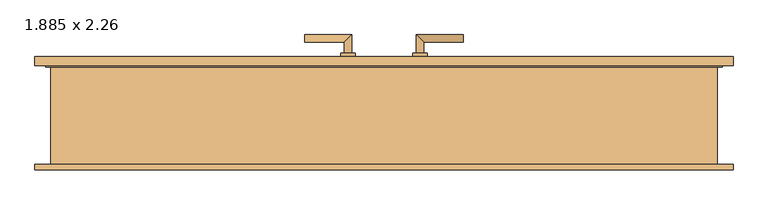
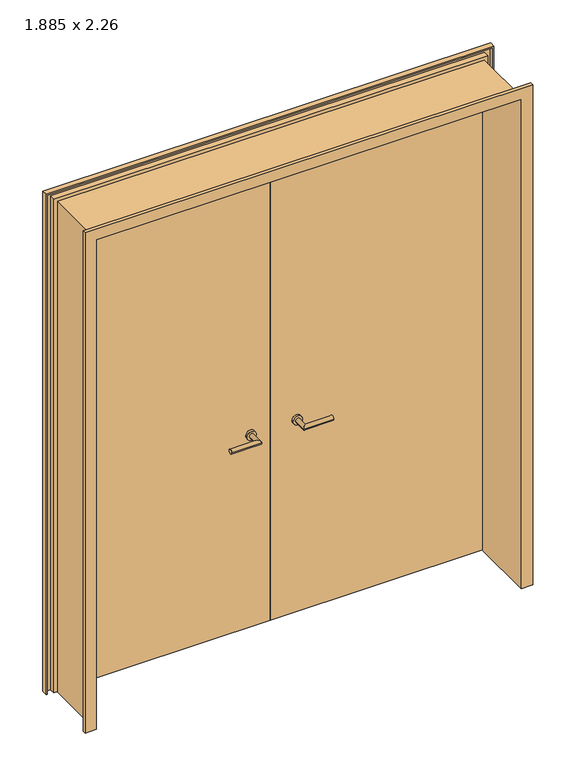
"""IFC4 building model written with IfcOpenShell, lengths in millimetres: door geometry, Drehflügel 2-flg - Stahlzarge : 1.885 x 2.26."""

from ifc_helpers import new_model, si_unit, point, frame, frame_2d, origin, place, context, project, spatial, polyline, circle_curve, ellipse_curve, trimmed, segment, composite_curve, outline, extrude, faceted_brep, source, transform, mapped, element, save
from ifc_brep_helpers import plane_surface, cylinder_surface, advanced_brep


def door_1_885_x_2_26_ea08af73(model_context):
    return source(origin(), model_context, "Body", "SolidModel", [
        advanced_brep(
        [(-90.0, 126.9346141, 1000.0), (-110.0, 126.9346141, 1000.0), (-110.0, 76.9346141, 1000.0), (-90.0, 56.9346141, 1000.0), (-220.0, 56.9346141, 1000.0), (-220.0, 76.9346141, 1000.0)],
        [
            (0, 1, circle_curve(frame((-100.0, 126.9346141, 1000.0), z_axis=(0.0, 1.0, 0.0), x_axis=(-1.0, 0.0, 0.0)), 10.0)),
            (1, 0, circle_curve(frame((-100.0, 126.9346141, 1000.0), z_axis=(0.0, 1.0, 0.0), x_axis=(-1.0, 0.0, 0.0)), 10.0)),
            (1, 2),
            (2, 3, ellipse_curve(frame((-100.0, 66.9346141, 1000.0), z_axis=(0.7071067811865385, 0.7071067811865565, 0.0), x_axis=(-0.7071067811865563, 0.7071067811865386, 0.0)), 14.1421356, 10.0)),
            (3, 0),
            (3, 2, ellipse_curve(frame((-100.0, 66.9346141, 1000.0), z_axis=(0.7071067811865385, 0.7071067811865565, 0.0), x_axis=(-0.7071067811865563, 0.7071067811865386, 0.0)), 14.1421356, 10.0)),
            (4, 5, circle_curve(frame((-220.0, 66.9346141, 1000.0), z_axis=(-1.0, 0.0, 0.0), x_axis=(0.0, 1.0, 0.0)), 10.0)),
            (5, 4, circle_curve(frame((-220.0, 66.9346141, 1000.0), z_axis=(-1.0, 0.0, 0.0), x_axis=(0.0, 1.0, 0.0)), 10.0)),
            (2, 5),
            (4, 3),
        ],
        [
            plane_surface(frame((-100.0, 126.9346141, -287.7526403), z_axis=(0.0, 1.0, 0.0), x_axis=(0.0, 0.0, 1.0))),
            cylinder_surface(frame((-100.0, 126.9346141, 1000.0), z_axis=(0.0, 1.0, 0.0), x_axis=(-1.0, 0.0, 0.0)), 10.0),
            plane_surface(frame((-220.0, 66.9346141, -287.7526403), z_axis=(-1.0, 0.0, 0.0), x_axis=(0.0, 0.0, 1.0))),
            cylinder_surface(frame((-100.0, 66.9346141, 1000.0), z_axis=(1.0, 0.0, 0.0), x_axis=(0.0, 1.0, 0.0)), 10.0),
        ],
        [
            (0, [[1, 2]]),
            (1, [[3, 4, 5, -2]]),
            (1, [[-5, 6, -3, -1]]),
            (2, [[7, 8]]),
            (3, [[9, -7, 10, -4]]),
            (3, [[-10, -8, -9, -6]]),
        ],
    ),
        advanced_brep(
        [(-110.0, 186.9346141, 1000.0), (-90.0, 186.9346141, 1000.0), (-90.0, 236.9346141, 1000.0), (-110.0, 216.9346141, 1000.0), (-220.0, 216.9346141, 1000.0), (-220.0, 236.9346141, 1000.0)],
        [
            (0, 1, circle_curve(frame((-100.0, 186.9346141, 1000.0), z_axis=(0.0, -1.0, 0.0), x_axis=(1.0, 0.0, 0.0)), 10.0)),
            (1, 0, circle_curve(frame((-100.0, 186.9346141, 1000.0), z_axis=(0.0, -1.0, 0.0), x_axis=(1.0, 0.0, 0.0)), 10.0)),
            (1, 2),
            (2, 3, ellipse_curve(frame((-100.0, 226.9346141, 1000.0), z_axis=(0.7071067811865475, -0.7071067811865475, 0.0), x_axis=(-0.7071067811865474, -0.7071067811865476, 0.0)), 14.1421356, 10.0)),
            (3, 0),
            (3, 2, ellipse_curve(frame((-100.0, 226.9346141, 1000.0), z_axis=(0.7071067811865475, -0.7071067811865475, 0.0), x_axis=(-0.7071067811865474, -0.7071067811865476, 0.0)), 14.1421356, 10.0)),
            (4, 5, circle_curve(frame((-220.0, 226.9346141, 1000.0), z_axis=(-1.0, 0.0, 0.0), x_axis=(0.0, 1.0, 0.0)), 10.0)),
            (5, 4, circle_curve(frame((-220.0, 226.9346141, 1000.0), z_axis=(-1.0, 0.0, 0.0), x_axis=(0.0, 1.0, 0.0)), 10.0)),
            (2, 5),
            (4, 3),
        ],
        [
            plane_surface(frame((-100.0, 186.9346141, -287.7526403), z_axis=(0.0, -1.0, 0.0), x_axis=(0.0, 0.0, 1.0))),
            cylinder_surface(frame((-100.0, 186.9346141, 1000.0), z_axis=(0.0, -1.0, 0.0), x_axis=(1.0, 0.0, 0.0)), 10.0),
            plane_surface(frame((-220.0, 226.9346141, -287.7526403), z_axis=(-1.0, 0.0, 0.0), x_axis=(0.0, 0.0, 1.0))),
            cylinder_surface(frame((-100.0, 226.9346141, 1000.0), z_axis=(1.0, 0.0, 0.0), x_axis=(0.0, 1.0, 0.0)), 10.0),
        ],
        [
            (0, [[1, 2]]),
            (1, [[3, 4, 5, -2]]),
            (1, [[-5, 6, -3, -1]]),
            (2, [[7, 8]]),
            (3, [[9, -7, 10, -4]]),
            (3, [[-10, -8, -9, -6]]),
        ],
    ),
        extrude(outline(composite_curve([segment(trimmed(circle_curve(frame_2d((1000.0, -100.0)), 20.0), [point((1000.0, -80.0))], [point((1000.0, -120.0))], False, "CARTESIAN"), True, "CONTINUOUS"), segment(trimmed(circle_curve(frame_2d((1000.0, -100.0)), 20.0), [point((1000.0, -120.0))], [point((1000.0, -80.0))], False, "CARTESIAN"), True, "CONTINUOUS")], self_intersect=False)), frame((0.0, 116.9346141, 0.0), z_axis=(0.0, 1.0, 0.0), x_axis=(0.0, 0.0, 1.0)), (0.0, 0.0, 1.0), 10.0),
        extrude(outline(composite_curve([segment(trimmed(circle_curve(frame_2d((1000.0, -100.0)), 20.0), [point((1000.0, -80.0))], [point((1000.0, -120.0))], False, "CARTESIAN"), True, "CONTINUOUS"), segment(trimmed(circle_curve(frame_2d((1000.0, -100.0)), 20.0), [point((1000.0, -120.0))], [point((1000.0, -80.0))], False, "CARTESIAN"), True, "CONTINUOUS")], self_intersect=False)), frame((0.0, 176.9346141, 0.0), z_axis=(0.0, 1.0, 0.0), x_axis=(0.0, 0.0, 1.0)), (0.0, 0.0, 1.0), 10.0),
        advanced_brep(
        [(90.0, 126.9346141, 1000.0), (110.0, 126.9346141, 1000.0), (90.0, 56.9346141, 1000.0), (110.0, 76.9346141, 1000.0), (220.0, 56.9346141, 1000.0), (220.0, 76.9346141, 1000.0)],
        [
            (0, 1, circle_curve(frame((100.0, 126.9346141, 1000.0), z_axis=(0.0, 1.0, 0.0), x_axis=(1.0, 0.0, 0.0)), 10.0)),
            (1, 0, circle_curve(frame((100.0, 126.9346141, 1000.0), z_axis=(0.0, 1.0, 0.0), x_axis=(1.0, 0.0, 0.0)), 10.0)),
            (0, 2),
            (2, 3, ellipse_curve(frame((100.0, 66.9346141, 1000.0), z_axis=(-0.7071067811865385, 0.7071067811865565, 0.0), x_axis=(0.7071067811865563, 0.7071067811865386, 0.0)), 14.1421356, 10.0)),
            (3, 1),
            (3, 2, ellipse_curve(frame((100.0, 66.9346141, 1000.0), z_axis=(-0.7071067811865385, 0.7071067811865565, 0.0), x_axis=(0.7071067811865563, 0.7071067811865386, 0.0)), 14.1421356, 10.0)),
            (4, 5, circle_curve(frame((220.0, 66.9346141, 1000.0), z_axis=(1.0, 0.0, 0.0), x_axis=(0.0, 1.0, 0.0)), 10.0)),
            (5, 4, circle_curve(frame((220.0, 66.9346141, 1000.0), z_axis=(1.0, 0.0, 0.0), x_axis=(0.0, 1.0, 0.0)), 10.0)),
            (2, 4),
            (5, 3),
        ],
        [
            plane_surface(frame((100.0, 126.9346141, -287.7526403), z_axis=(0.0, 1.0, 0.0), x_axis=(0.0, 0.0, 1.0))),
            cylinder_surface(frame((100.0, 126.9346141, 1000.0), z_axis=(0.0, 1.0, 0.0), x_axis=(1.0, 0.0, 0.0)), 10.0),
            plane_surface(frame((220.0, 66.9346141, -287.7526403), z_axis=(1.0, 0.0, 0.0), x_axis=(0.0, 0.0, 1.0))),
            cylinder_surface(frame((100.0, 66.9346141, 1000.0), z_axis=(-1.0, 0.0, 0.0), x_axis=(0.0, 1.0, 0.0)), 10.0),
        ],
        [
            (0, [[1, 2]]),
            (1, [[-1, 3, 4, 5]]),
            (1, [[-2, -5, 6, -3]]),
            (2, [[7, 8]]),
            (3, [[-4, 9, -8, 10]]),
            (3, [[-6, -10, -7, -9]]),
        ],
    ),
        advanced_brep(
        [(110.0, 186.9346141, 1000.0), (90.0, 186.9346141, 1000.0), (110.0, 216.9346141, 1000.0), (90.0, 236.9346141, 1000.0), (220.0, 216.9346141, 1000.0), (220.0, 236.9346141, 1000.0)],
        [
            (0, 1, circle_curve(frame((100.0, 186.9346141, 1000.0), z_axis=(0.0, -1.0, 0.0), x_axis=(-1.0, 0.0, 0.0)), 10.0)),
            (1, 0, circle_curve(frame((100.0, 186.9346141, 1000.0), z_axis=(0.0, -1.0, 0.0), x_axis=(-1.0, 0.0, 0.0)), 10.0)),
            (0, 2),
            (2, 3, ellipse_curve(frame((100.0, 226.9346141, 1000.0), z_axis=(-0.7071067811865475, -0.7071067811865475, 0.0), x_axis=(0.7071067811865474, -0.7071067811865476, 0.0)), 14.1421356, 10.0)),
            (3, 1),
            (3, 2, ellipse_curve(frame((100.0, 226.9346141, 1000.0), z_axis=(-0.7071067811865475, -0.7071067811865475, 0.0), x_axis=(0.7071067811865474, -0.7071067811865476, 0.0)), 14.1421356, 10.0)),
            (4, 5, circle_curve(frame((220.0, 226.9346141, 1000.0), z_axis=(1.0, 0.0, 0.0), x_axis=(0.0, 1.0, 0.0)), 10.0)),
            (5, 4, circle_curve(frame((220.0, 226.9346141, 1000.0), z_axis=(1.0, 0.0, 0.0), x_axis=(0.0, 1.0, 0.0)), 10.0)),
            (2, 4),
            (5, 3),
        ],
        [
            plane_surface(frame((100.0, 186.9346141, -287.7526403), z_axis=(0.0, -1.0, 0.0), x_axis=(0.0, 0.0, 1.0))),
            cylinder_surface(frame((100.0, 186.9346141, 1000.0), z_axis=(0.0, -1.0, 0.0), x_axis=(-1.0, 0.0, 0.0)), 10.0),
            plane_surface(frame((220.0, 226.9346141, -287.7526403), z_axis=(1.0, 0.0, 0.0), x_axis=(0.0, 0.0, 1.0))),
            cylinder_surface(frame((100.0, 226.9346141, 1000.0), z_axis=(-1.0, 0.0, 0.0), x_axis=(0.0, 1.0, 0.0)), 10.0),
        ],
        [
            (0, [[1, 2]]),
            (1, [[-1, 3, 4, 5]]),
            (1, [[-2, -5, 6, -3]]),
            (2, [[7, 8]]),
            (3, [[-4, 9, -8, 10]]),
            (3, [[-6, -10, -7, -9]]),
        ],
    ),
        extrude(outline(composite_curve([segment(trimmed(circle_curve(frame_2d((1000.0, 100.0)), 20.0), [point((1000.0, 80.0))], [point((1000.0, 120.0))], False, "CARTESIAN"), True, "CONTINUOUS"), segment(trimmed(circle_curve(frame_2d((1000.0, 100.0)), 20.0), [point((1000.0, 120.0))], [point((1000.0, 80.0))], False, "CARTESIAN"), True, "CONTINUOUS")], self_intersect=False)), frame((0.0, 116.9346141, 0.0), z_axis=(0.0, 1.0, 0.0), x_axis=(0.0, 0.0, 1.0)), (0.0, 0.0, 1.0), 10.0),
        extrude(outline(composite_curve([segment(trimmed(circle_curve(frame_2d((1000.0, 100.0)), 20.0), [point((1000.0, 80.0))], [point((1000.0, 120.0))], False, "CARTESIAN"), True, "CONTINUOUS"), segment(trimmed(circle_curve(frame_2d((1000.0, 100.0)), 20.0), [point((1000.0, 120.0))], [point((1000.0, 80.0))], False, "CARTESIAN"), True, "CONTINUOUS")], self_intersect=False)), frame((0.0, 176.9346141, 0.0), z_axis=(0.0, 1.0, 0.0), x_axis=(0.0, 0.0, 1.0)), (0.0, 0.0, 1.0), 10.0),
        extrude(outline(polyline([(0.0, 151.9346141), (-932.5, 151.9346141), (-932.5, 176.9346141), (0.0, 176.9346141), (0.0, 151.9346141)])), frame((0.0, 0.0, 100.0), z_axis=(0.0, 0.0, 1.0), x_axis=(1.0, 0.0, 0.0)), (0.0, 0.0, 1.0), 2250.0),
        extrude(outline(polyline([(932.5, 151.9346141), (0.0, 151.9346141), (0.0, 176.9346141), (932.5, 176.9346141), (932.5, 151.9346141)])), frame((0.0, 0.0, 100.0), z_axis=(0.0, 0.0, 1.0), x_axis=(1.0, 0.0, 0.0)), (0.0, 0.0, 1.0), 2250.0),
        faceted_brep([(967.0, -138.0653859, 100.0), (917.5, -138.0653859, 100.0), (917.5, 151.9346141, 100.0), (932.5, 151.9346141, 100.0), (932.5, 176.9346141, 100.0), (967.0, 176.9346141, 100.0), (967.0, 151.9346141, 100.0), (962.0, 151.9346141, 100.0), (962.0, 171.9346141, 100.0), (937.5, 171.9346141, 100.0), (937.5, 146.9346141, 100.0), (922.5, 146.9346141, 100.0), (922.5, -133.0653859, 100.0), (962.0, -133.0653859, 100.0), (962.0, -123.0653859, 100.0), (967.0, -123.0653859, 100.0), (967.0, -138.0653859, 2384.5), (-967.0, -138.0653859, 2384.5), (-967.0, -138.0653859, 100.0), (-917.5, -138.0653859, 100.0), (-917.5, -138.0653859, 2335.0), (917.5, -138.0653859, 2335.0), (917.5, 151.9346141, 2335.0), (-917.5, 151.9346141, 2335.0), (-917.5, 151.9346141, 100.0), (-932.5, 151.9346141, 100.0), (-932.5, 151.9346141, 2350.0), (932.5, 151.9346141, 2350.0), (932.5, 176.9346141, 2350.0), (-932.5, 176.9346141, 2350.0), (-932.5, 176.9346141, 100.0), (-967.0, 176.9346141, 100.0), (-967.0, 176.9346141, 2384.5), (967.0, 176.9346141, 2384.5), (967.0, 151.9346141, 2384.5), (-967.0, 151.9346141, 2384.5), (-967.0, 151.9346141, 100.0), (-962.0, 151.9346141, 100.0), (-962.0, 151.9346141, 2379.5), (962.0, 151.9346141, 2379.5), (962.0, 171.9346141, 2379.5), (-962.0, 171.9346141, 2379.5), (-962.0, 171.9346141, 100.0), (-937.5, 171.9346141, 100.0), (-937.5, 171.9346141, 2355.0), (937.5, 171.9346141, 2355.0), (937.5, 146.9346141, 2355.0), (-937.5, 146.9346141, 2355.0), (-937.5, 146.9346141, 100.0), (-922.5, 146.9346141, 100.0), (-922.5, 146.9346141, 2340.0), (922.5, 146.9346141, 2340.0), (922.5, -133.0653859, 2340.0), (-922.5, -133.0653859, 2340.0), (-922.5, -133.0653859, 100.0), (-962.0, -133.0653859, 100.0), (-962.0, -133.0653859, 2379.5), (962.0, -133.0653859, 2379.5), (962.0, -123.0653859, 2379.5), (-962.0, -123.0653859, 2379.5), (-962.0, -123.0653859, 100.0), (-967.0, -123.0653859, 100.0), (-967.0, -123.0653859, 2384.5), (967.0, -123.0653859, 2384.5)], [[[0, 1, 2, 3, 4, 5, 6, 7, 8, 9, 10, 11, 12, 13, 14, 15]], [[1, 0, 16, 17, 18, 19, 20, 21]], [[2, 1, 21, 22]], [[3, 2, 22, 23, 24, 25, 26, 27]], [[4, 3, 27, 28]], [[5, 4, 28, 29, 30, 31, 32, 33]], [[6, 5, 33, 34]], [[7, 6, 34, 35, 36, 37, 38, 39]], [[8, 7, 39, 40]], [[9, 8, 40, 41, 42, 43, 44, 45]], [[10, 9, 45, 46]], [[11, 10, 46, 47, 48, 49, 50, 51]], [[12, 11, 51, 52]], [[13, 12, 52, 53, 54, 55, 56, 57]], [[14, 13, 57, 58]], [[15, 14, 58, 59, 60, 61, 62, 63]], [[0, 15, 63, 16]], [[17, 62, 61, 18]], [[18, 61, 60, 55, 54, 49, 48, 43, 42, 37, 36, 31, 30, 25, 24, 19]], [[23, 20, 19, 24]], [[29, 26, 25, 30]], [[35, 32, 31, 36]], [[41, 38, 37, 42]], [[47, 44, 43, 48]], [[53, 50, 49, 54]], [[59, 56, 55, 60]], [[22, 21, 20, 23]], [[28, 27, 26, 29]], [[34, 33, 32, 35]], [[40, 39, 38, 41]], [[46, 45, 44, 47]], [[52, 51, 50, 53]], [[58, 57, 56, 59]], [[16, 63, 62, 17]]]),
    ])


if __name__ == "__main__":
    model = new_model("IFC4")
    model_context = context("Model", 3, world=origin())
    ifc_project = project(units=[si_unit("LENGTHUNIT", "METRE", prefix="MILLI")], contexts=[model_context])
    site = spatial("IfcSite", under=ifc_project)
    building = spatial("IfcBuilding", under=site)
    placement = place(None, origin())
    door_1_885_x_2_26_shape = door_1_885_x_2_26_ea08af73(model_context)
    element("IfcDoor", 1, ObjectType="Drehflügel 2-flg - Stahlzarge : 1.885 x 2.26", at=placement, inside=building, context=model_context, shape_type="MappedRepresentation", body=[
        mapped(door_1_885_x_2_26_shape, transform((0.0, 0.0, 0.0), x_axis=(1.0, 0.0, 0.0), y_axis=(0.0, 1.0, 0.0), z_axis=(0.0, 0.0, 1.0))),
    ])
    save(model, "model.ifc")

# Revit data of these elements
# Type "Drehflügel 2-flg - Stahlzarge : 1.885 x 2.26"
#   Construction Type Id = "DOOR"
#   Type Mark = "19"
#   Operation = "DoubleDoorSingleSwing"
#   Keynote = "16.03"
#   Analytic Construction = "Hölzern"
#   Thermal Resistance (R) = 0.270117 (m²·K)/W
#   Heat Transfer Coefficient (U) = 2.1944 W/(m²·K)
#   Rough Width = 1.885 m
#   Rough Height [instance default] = 2.360 m
#   Höhe Türgriff = 0.900 m
#   Height = 2.260 m
#   Fußbodenaufbau [instance default] = 0.100 m
#   Width = 1.885 m
#   Sichtbarkeit Sturzlinien [instance default] = yes
#   Türgriff auswählen [instance default] = element 219327
#   Türgriff [instance default] = none
#   Türflügel [instance default] = none
#   Rahmen/Pfosten [instance default] = Metall - Lackiert - Grau
#   Visual Light Transmittance = 0
#   Solar Heat Gain Coefficient = 0
#   Function = (empty or 0)
#   Wall Closure = (empty or 0)
# Element 1 (IfcDoor, "Drehflügel 2-flg - Stahlzarge : 1.885 x 2.26")
#   Materials on its faces: "Metall - Chrom", "Metall - Lackiert - Grau", "Holz - Birke"
# Materials
#   "Metall - Lackiert - Grau": class "Farbe 1", colour RGB 98 98 98, transparency 0, Cost = 0
#   "Metall - Chrom": class "Metall", colour RGB 247 247 247, transparency 0, Cost = 0
#   "Holz - Birke": class "Holz", colour RGB 213 164 103, transparency 0, Cost = 0
